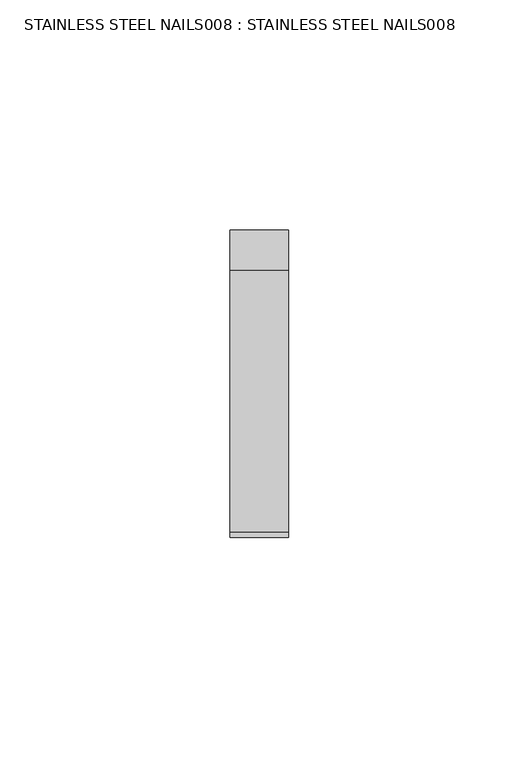
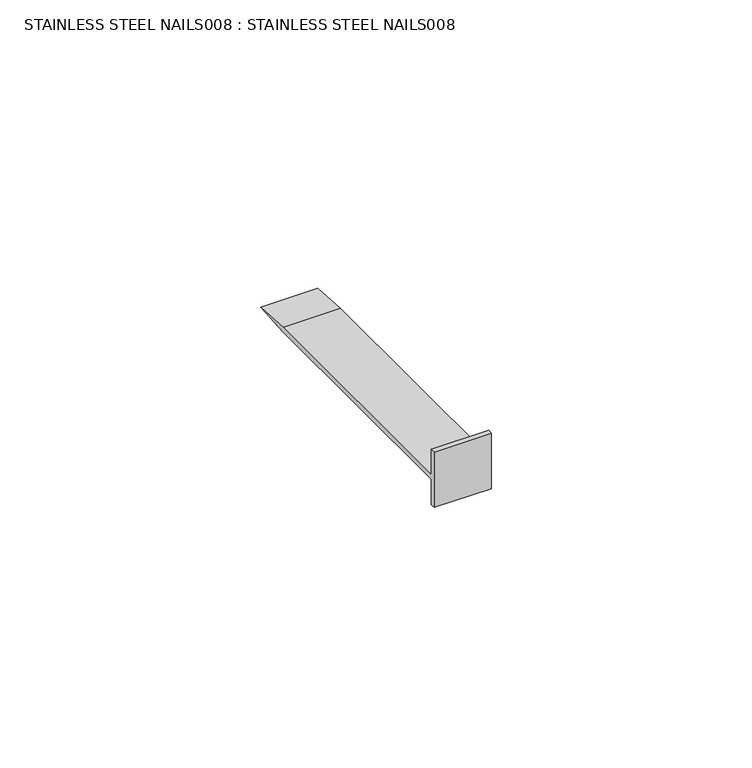
"""IFC4 building model written with IfcOpenShell, lengths in millimetres: proxy geometry, STAINLESS STEEL NAILS008 : STAINLESS STEEL NAILS008."""

from ifc_helpers import new_model, si_unit, frame, origin, place, context, project, spatial, polyline, outline, extrude, source, transform, mapped, element, save


def stainless_steel_nails008_stainless_steel_nails008_ed18b8cf(model_context):
    return source(origin(), model_context, "Body", "SweptSolid", [
        extrude(outline(polyline([(-5577.378205, 40134.3588724), (-5577.378205, 40147.3572563), (-5576.2950063, 40147.3572563), (-5576.2950063, 40141.3996637), (-5519.393468, 40141.3996637), (-5510.7278788, 40140.8591651), (-5519.4110792, 40140.316465), (-5576.2950063, 40140.316465), (-5576.2950063, 40134.3588724), (-5577.378205, 40134.3588724)])), frame((14383.0178845, 0.0, 0.0), z_axis=(1.0, 0.0, 0.0), x_axis=(0.0, 1.0, 0.0)), (0.0, 0.0, 1.0), 12.7),
    ])


if __name__ == "__main__":
    model = new_model("IFC4")
    model_context = context("Model", 3, world=origin())
    ifc_project = project(units=[si_unit("LENGTHUNIT", "METRE", prefix="MILLI")], contexts=[model_context])
    site = spatial("IfcSite", under=ifc_project)
    building = spatial("IfcBuilding", under=site)
    placement = place(None, origin())
    stainless_steel_nails008_stainless_steel_nails008_shape = stainless_steel_nails008_stainless_steel_nails008_ed18b8cf(model_context)
    element("IfcBuildingElementProxy", 1, Name="STAINLESS STEEL NAILS008 : STAINLESS STEEL NAILS008", ObjectType="STAINLESS STEEL NAILS008 : STAINLESS STEEL NAILS008", at=placement, inside=building, context=model_context, shape_type="MappedRepresentation", body=[
        mapped(stainless_steel_nails008_stainless_steel_nails008_shape, transform((0.0, 0.0, 0.0), x_axis=(1.0, 0.0, 0.0), y_axis=(0.0, 1.0, 0.0), z_axis=(0.0, 0.0, 1.0))),
    ])
    save(model, "model.ifc")

# Revit data of these elements
# Type "STAINLESS STEEL NAILS008 : STAINLESS STEEL NAILS008"
#   NameOverride = "STAINLESS STEEL NAILS008"
# Element 1 (IfcBuildingElementProxy, "STAINLESS STEEL NAILS008 : STAINLESS STEEL NAILS008")
#   Materials on its faces: "1 3/4\" STAINLESS STEEL RINGSHANK 5D COMMON NAILS @ 4\" (101.6MM) O.C. FIRESTONE PROVIDED MAX., 1/2\" STAGGERED"
# Materials
#   "1 3/4\" STAINLESS STEEL RINGSHANK 5D COMMON NAILS @ 4\" (101.6MM) O.C. FIRESTONE PROVIDED MAX., 1/2\" STAGGERED": class "Unassigned", colour RGB 255 255 255, transparency 0
